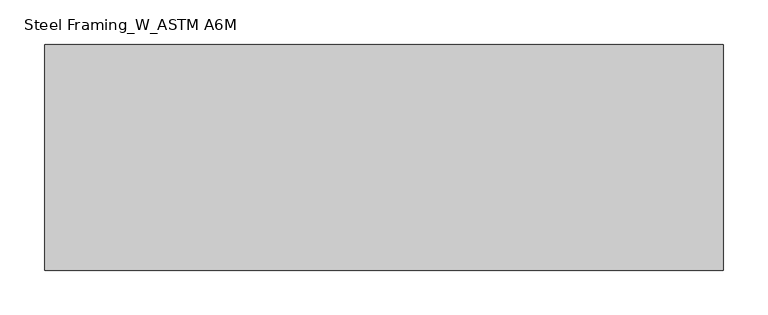
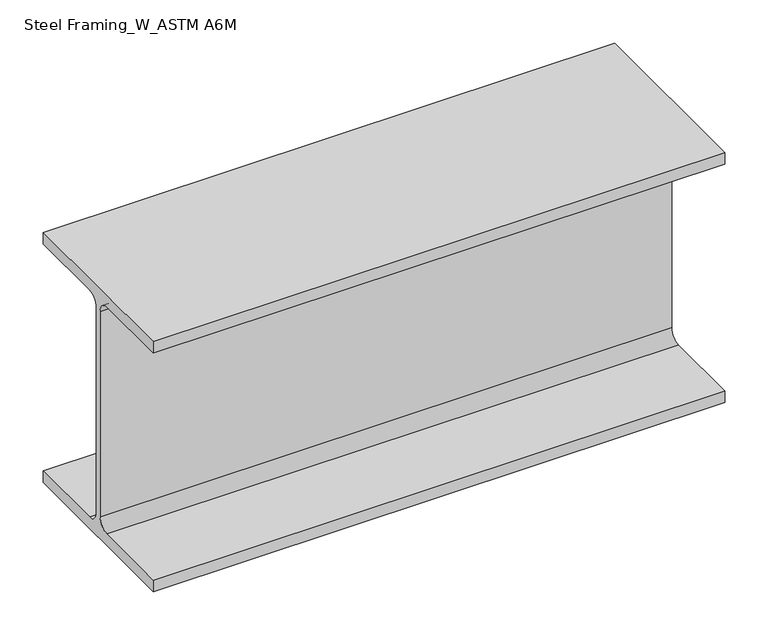
"""IFC4 building model written with IfcOpenShell, lengths in millimetres: beam geometry, Steel Framing_W_ASTM A6M : H_SB_AR_S02_W360x91_B3."""

import ifcopenshell
import ifcopenshell.guid

model = None  # the IFC model being written
_history = None  # IfcOwnerHistory: only IFC2X3 demands one
_inside = {}  # id of a spatial element -> (the spatial element, [elements in it])
_under = {}  # id of a project, library or spatial element -> (it, [spatial elements below it])
_declared = {}  # id of a project -> (the project, [libraries it declares])
_typed = {}  # id of a type object -> (the type object, [elements of that type])
_made_of = {}  # id of a material, layer set ... -> (it, [elements and type objects made of it])


def new_model(schema):
    """Start an empty IFC model of exactly this schema.

    Asked for "IFC4X3", IfcOpenShell would pick the latest addendum, in which some entities
    have other attributes; the version numbers below select the first issue.
    IFC2X3 requires an IfcOwnerHistory on every rooted entity: one is made here for all.
    """
    global model, _history
    if schema == "IFC4X3":
        model = ifcopenshell.file(schema_version=(4, 3, 0, 0))
    else:
        model = ifcopenshell.file(schema=schema)
    _inside.clear()
    _under.clear()
    _declared.clear()
    _typed.clear()
    _made_of.clear()
    _history = None
    if model.schema == "IFC2X3":
        org = make("IfcOrganization", Name="unknown")
        user = make(
            "IfcPersonAndOrganization",
            ThePerson=make("IfcPerson", FamilyName="unknown"),
            TheOrganization=org,
        )
        app = make(
            "IfcApplication",
            ApplicationDeveloper=org,
            Version="unknown",
            ApplicationFullName="unknown",
            ApplicationIdentifier="unknown",
        )
        _history = make(
            "IfcOwnerHistory",
            OwningUser=user,
            OwningApplication=app,
            ChangeAction="ADDED",
            CreationDate=0,
        )
    return model


def make(cls, **values):
    """One entity of the class cls with the attributes given. An attribute that is None is left unset."""
    return model.create_entity(
        cls, **{name: value for name, value in values.items() if value is not None}
    )


def rooted(cls, **values):
    """An entity with a GlobalId (a new one), such as an element, a storey or a relation."""
    return make(cls, GlobalId=ifcopenshell.guid.new(), OwnerHistory=_history, **values)


def si_unit(unit_type, name, prefix=None):
    """IfcSIUnit, for example si_unit("LENGTHUNIT", "METRE", prefix="MILLI")."""
    return make("IfcSIUnit", UnitType=unit_type, Prefix=prefix, Name=name)


def assignment(units):
    """IfcUnitAssignment: the units of a project."""
    return None if units is None else make("IfcUnitAssignment", Units=units)


def point(xyz):
    """IfcCartesianPoint."""
    return None if xyz is None else make("IfcCartesianPoint", Coordinates=xyz)


def direction(xyz):
    """IfcDirection."""
    return None if xyz is None else make("IfcDirection", DirectionRatios=xyz)


def frame(location, z_axis=None, x_axis=None):
    """IfcAxis2Placement3D, a coordinate frame: its origin and axes. An axis left out is left unset."""
    return make(
        "IfcAxis2Placement3D",
        Location=point(location),
        Axis=direction(z_axis),
        RefDirection=direction(x_axis),
    )


def frame_2d(location, x_axis=None):
    """IfcAxis2Placement2D, a coordinate frame in the plane: its origin and x axis."""
    return make(
        "IfcAxis2Placement2D", Location=point(location), RefDirection=direction(x_axis)
    )


def origin():
    """The frame at (0, 0, 0) with its axes left unset."""
    return frame((0.0, 0.0, 0.0))


def place(relative_to, where):
    """IfcLocalPlacement: puts the frame where relative to a parent placement (None: the world)."""
    return make(
        "IfcLocalPlacement", PlacementRelTo=relative_to, RelativePlacement=where
    )


def context(
    kind, dimensions, precision=None, world=None, true_north=None, identifier=None
):
    """IfcGeometricRepresentationContext, for example the 3D "Model" context."""
    return make(
        "IfcGeometricRepresentationContext",
        ContextIdentifier=identifier,
        ContextType=kind,
        CoordinateSpaceDimension=dimensions,
        Precision=precision,
        WorldCoordinateSystem=world,
        TrueNorth=true_north,
    )


def project(units=None, contexts=None):
    """IfcProject with its units and contexts."""
    return rooted(
        "IfcProject",
        Name="project",
        RepresentationContexts=contexts,
        UnitsInContext=assignment(units),
    )


def spatial(cls, under=None, at=None, **own):
    """A site, building, storey or space (cls), placed at a placement, below another one or the project."""
    s = rooted(cls, ObjectPlacement=at, **own)
    if under is not None:
        _under.setdefault(under.id(), (under, []))[1].append(s)
    return s


def polyline(points):
    """IfcPolyline through the points."""
    return make("IfcPolyline", Points=[point(p) for p in points])


def circle_curve(where, radius):
    """IfcCircle in the frame where."""
    return make("IfcCircle", Position=where, Radius=radius)


def trimmed(basis, trim1, trim2, sense, master):
    """IfcTrimmedCurve: the piece of a basis curve between two trims."""
    return make(
        "IfcTrimmedCurve",
        BasisCurve=basis,
        Trim1=trim1,
        Trim2=trim2,
        SenseAgreement=sense,
        MasterRepresentation=master,
    )


def segment(curve, same_sense, transition):
    """IfcCompositeCurveSegment."""
    return make(
        "IfcCompositeCurveSegment",
        Transition=transition,
        SameSense=same_sense,
        ParentCurve=curve,
    )


def composite_curve(segments, self_intersect=None):
    """IfcCompositeCurve: segments joined end to end."""
    return make("IfcCompositeCurve", Segments=segments, SelfIntersect=self_intersect)


def outline(outer, holes=None, kind="AREA"):
    """IfcArbitraryClosedProfileDef: a profile drawn as a closed curve; with holes, ...WithVoids."""
    if holes is None:
        return make("IfcArbitraryClosedProfileDef", ProfileType=kind, OuterCurve=outer)
    return make(
        "IfcArbitraryProfileDefWithVoids",
        ProfileType=kind,
        OuterCurve=outer,
        InnerCurves=holes,
    )


def extrude(swept, where, along, depth):
    """IfcExtrudedAreaSolid: the profile swept, set in the frame where, extruded along a direction by depth."""
    return make(
        "IfcExtrudedAreaSolid",
        SweptArea=swept,
        Position=where,
        ExtrudedDirection=direction(along),
        Depth=depth,
    )


def shape(context_of_items, identifier, shape_type, items):
    """IfcShapeRepresentation: the items that make up one representation, for example the "Body"."""
    return make(
        "IfcShapeRepresentation",
        ContextOfItems=context_of_items,
        RepresentationIdentifier=identifier,
        RepresentationType=shape_type,
        Items=items,
    )


def source(mapping_origin, context_of_items, identifier, shape_type, items):
    """IfcRepresentationMap: a shape defined once, which mapped items show again and again."""
    return make(
        "IfcRepresentationMap",
        MappingOrigin=mapping_origin,
        MappedRepresentation=shape(context_of_items, identifier, shape_type, items),
    )


def transform(
    local_origin,
    x_axis=None,
    y_axis=None,
    z_axis=None,
    scale=None,
    scale2=None,
    scale3=None,
    uniform=True,
):
    """IfcCartesianTransformationOperator3D, or its non-uniform kind. x_axis, y_axis, z_axis: its Axis1, 2, 3."""
    if uniform:
        return make(
            "IfcCartesianTransformationOperator3D",
            Axis1=direction(x_axis),
            Axis2=direction(y_axis),
            LocalOrigin=point(local_origin),
            Scale=scale,
            Axis3=direction(z_axis),
        )
    return make(
        "IfcCartesianTransformationOperator3DnonUniform",
        Axis1=direction(x_axis),
        Axis2=direction(y_axis),
        LocalOrigin=point(local_origin),
        Scale=scale,
        Axis3=direction(z_axis),
        Scale2=scale2,
        Scale3=scale3,
    )


def mapped(mapping_source, mapping_target):
    """IfcMappedItem: shows the shape of a source again, moved by a transform."""
    return make(
        "IfcMappedItem", MappingSource=mapping_source, MappingTarget=mapping_target
    )


def made_of(thing, what):
    """Note that an element or type object is made of a material, layer set ...; save() writes the relation."""
    if what is not None:
        _made_of.setdefault(what.id(), (what, []))[1].append(thing)
    return thing


def element(
    cls,
    number,
    at=None,
    inside=None,
    cuts=None,
    type_object=None,
    material=None,
    context=None,
    identifier="Body",
    shape_type=None,
    held_by="IfcProductDefinitionShape",
    body=None,
    shapes=None,
    **own,
):
    """One element of the class cls, such as IfcWall. Its Tag is "e" and its number.

    at: its placement. inside: the storey or other place that contains it. cuts: it is an
    opening in that element (IfcRelVoidsElement). A single representation is given by context,
    identifier, shape_type and body (its items); several are given by shapes. held_by: the class
    of the entity that holds the representations. save() writes the other relations.
    """
    e = rooted(cls, Tag="e%d" % number, ObjectPlacement=at, **own)
    if body is not None:
        shapes = [shape(context, identifier, shape_type, body)]
    if shapes is not None:
        e.Representation = make(held_by, Representations=shapes)
    if inside is not None:
        _inside.setdefault(inside.id(), (inside, []))[1].append(e)
    if cuts is not None:
        rooted(
            "IfcRelVoidsElement", RelatingBuildingElement=cuts, RelatedOpeningElement=e
        )
    if type_object is not None:
        _typed.setdefault(type_object.id(), (type_object, []))[1].append(e)
    return made_of(e, material)


def aggregate(whole, parts):
    """IfcRelAggregates: a whole, such as a stair, and the parts it consists of."""
    return rooted("IfcRelAggregates", RelatingObject=whole, RelatedObjects=parts)


def save(model, path):
    """Write the relations noted so far, then the file.

    IfcRelAggregates (storeys below a building ...), IfcRelContainedInSpatialStructure (elements
    in a storey), IfcRelDefinesByType, IfcRelAssociatesMaterial and IfcRelDeclares: one each for
    every whole, place, type object, material and project.
    """
    for whole, parts in _under.values():
        aggregate(whole, parts)
    for where, things in _inside.values():
        rooted(
            "IfcRelContainedInSpatialStructure",
            RelatedElements=things,
            RelatingStructure=where,
        )
    for kind, things in _typed.values():
        rooted("IfcRelDefinesByType", RelatedObjects=things, RelatingType=kind)
    for what, things in _made_of.values():
        rooted("IfcRelAssociatesMaterial", RelatedObjects=things, RelatingMaterial=what)
    for by, libraries in _declared.values():
        rooted("IfcRelDeclares", RelatingContext=by, RelatedDefinitions=libraries)
    model.write(path)


def steel_framing_w_astm_a6m_e4d07942(model_context):
    return source(origin(), model_context, "Body", "SweptSolid", [
        extrude(outline(composite_curve([segment(polyline([(127.0, -160.1), (127.0, -176.5), (-127.0, -176.5), (-127.0, -160.1), (-19.865, -160.1)]), True, "CONTINUOUS"), segment(trimmed(circle_curve(frame_2d((-19.865, -145.0)), 15.1), [point((-19.865, -160.1))], [point((-4.765, -145.0))], True, "CARTESIAN"), True, "CONTINUOUS"), segment(polyline([(-4.765, -145.0), (-4.765, 145.0)]), True, "CONTINUOUS"), segment(trimmed(circle_curve(frame_2d((-19.865, 145.0)), 15.1), [point((-4.765, 145.0))], [point((-19.865, 160.1))], True, "CARTESIAN"), True, "CONTINUOUS"), segment(polyline([(-19.865, 160.1), (-127.0, 160.1), (-127.0, 176.5), (127.0, 176.5), (127.0, 160.1), (19.865, 160.1)]), True, "CONTINUOUS"), segment(trimmed(circle_curve(frame_2d((19.865, 145.0)), 15.1), [point((19.865, 160.1))], [point((4.765, 145.0))], True, "CARTESIAN"), True, "CONTINUOUS"), segment(polyline([(4.765, 145.0), (4.765, -145.0)]), True, "CONTINUOUS"), segment(trimmed(circle_curve(frame_2d((19.865, -145.0)), 15.1), [point((4.765, -145.0))], [point((19.865, -160.1))], True, "CARTESIAN"), True, "CONTINUOUS"), segment(polyline([(19.865, -160.1), (127.0, -160.1)]), True, "CONTINUOUS")], self_intersect=False)), frame((-360.3, 0.0, 0.0), z_axis=(1.0, 0.0, 0.0), x_axis=(0.0, 1.0, 0.0)), (0.0, 0.0, 1.0), 762.1),
    ])


if __name__ == "__main__":
    model = new_model("IFC4")
    model_context = context("Model", 3, world=origin())
    ifc_project = project(units=[si_unit("LENGTHUNIT", "METRE", prefix="MILLI")], contexts=[model_context])
    site = spatial("IfcSite", under=ifc_project)
    building = spatial("IfcBuilding", under=site)
    placement = place(None, origin())
    steel_framing_w_astm_a6m_shape = steel_framing_w_astm_a6m_e4d07942(model_context)
    element("IfcBeam", 1, ObjectType="Steel Framing_W_ASTM A6M : H_SB_AR_S02_W360x91_B3", at=placement, inside=building, context=model_context, shape_type="MappedRepresentation", body=[
        mapped(steel_framing_w_astm_a6m_shape, transform((0.0, 0.0, 0.0), x_axis=(1.0, 0.0, 0.0), y_axis=(0.0, 1.0, 0.0), z_axis=(0.0, 0.0, 1.0))),
    ])
    save(model, "model.ifc")

# Revit data of these elements
# Type "Steel Framing_W_ASTM A6M : H_SB_AR_S02_W360x91_B3"
#   Type Mark = "B3"
#   Section Name Key = "W14x61"
#   Width = 25.4 cm
#   Web Thickness = 0.953 cm
#   Web Fillet = 1.51 cm
#   Warping Constant = 1260000.0 cm⁶
#   Torsional Moment of Inertia = 91.20 cm⁴
#   Section Area = 115.0 cm²
#   Plastic Modulus weak axis = 537.0 cm³
#   Plastic Modulus strong axis = 1670.0 cm³
#   Perimeter = 1.68 m²/m
#   Nominal Weight = 91.00 kgf/m
#   Moment of Inertia weak axis = 4450.00 cm⁴
#   Moment of Inertia strong axis = 26600.00 cm⁴
#   Height = 35.3 cm
#   Flange Thickness = 1.64 cm
#   Elastic Modulus weak axis = 352.0 cm³
#   Elastic Modulus strong axis = 1510.0 cm³
#   Centroid Vertical = 17.65 cm
#   Centroid Horizontal = 12.7 cm
#   Length [instance default] = 1500 mm
#   Structural Material [instance default] = Steel, 45-345
#   Bolt Spacing = 0
#   Assembly Code = ""
# Element 1 (IfcBeam, "Steel Framing_W_ASTM A6M : H_SB_AR_S02_W360x91_B3")
#   Materials on its faces: "Steel, 45-345"
# Materials
#   "Steel, 45-345": class "Metal", colour RGB 189 187 185, transparency 0, Description = "Steel 345 MPa", Cost = 0
